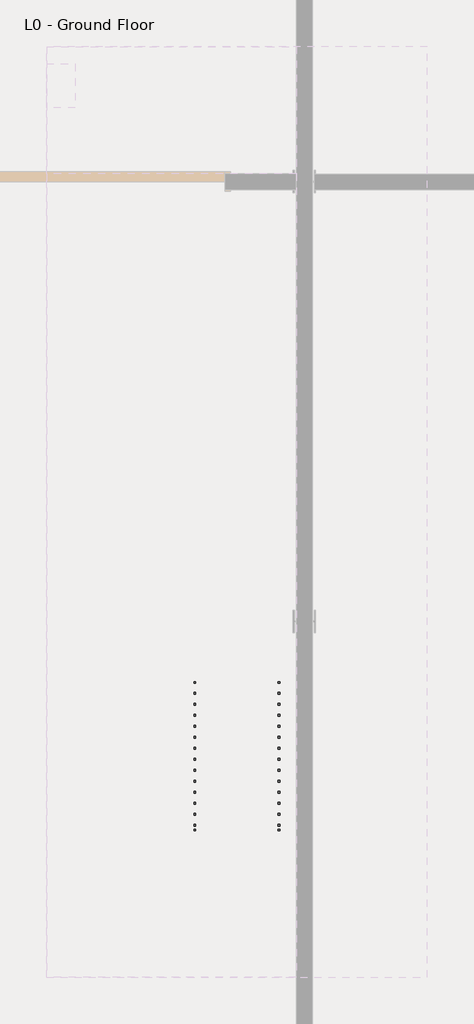
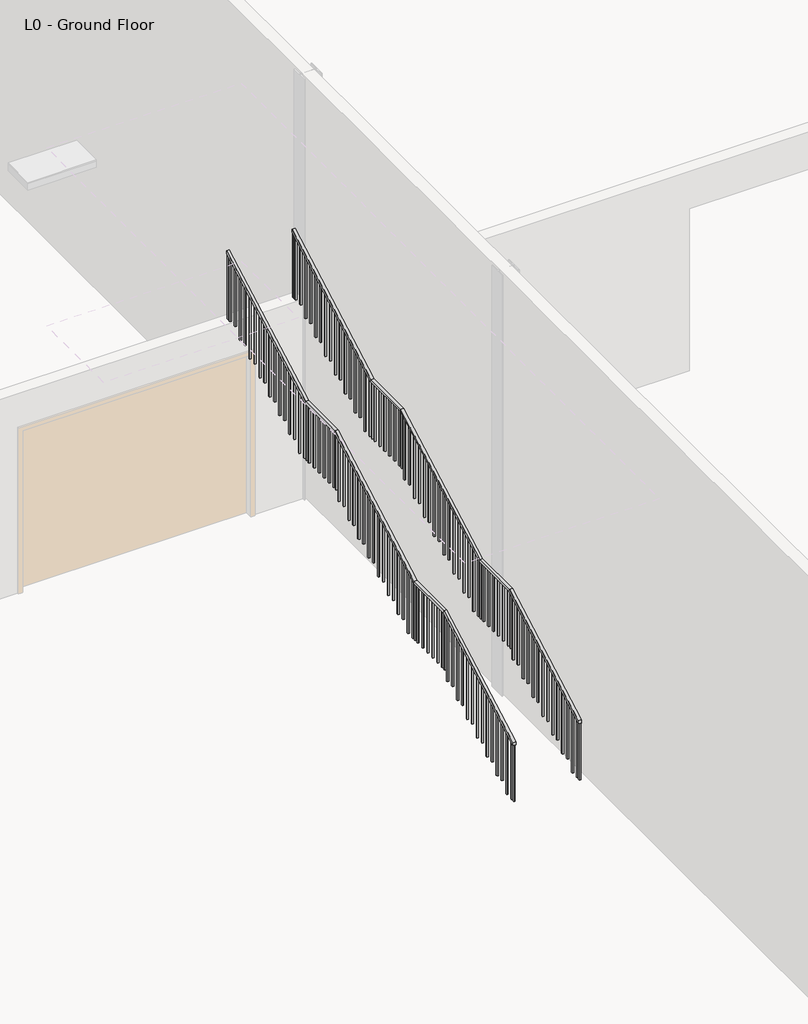
# One storey, part 9 of 14: 2 railings.
"""IFC4 building model written with IfcOpenShell, lengths in millimetres."""

import ifcopenshell
import ifcopenshell.guid

model = None  # the IFC model being written
_history = None  # IfcOwnerHistory: only IFC2X3 demands one
_inside = {}  # id of a spatial element -> (the spatial element, [elements in it])
_under = {}  # id of a project, library or spatial element -> (it, [spatial elements below it])
_declared = {}  # id of a project -> (the project, [libraries it declares])
_typed = {}  # id of a type object -> (the type object, [elements of that type])
_made_of = {}  # id of a material, layer set ... -> (it, [elements and type objects made of it])


def new_model(schema):
    """Start an empty IFC model of exactly this schema.

    Asked for "IFC4X3", IfcOpenShell would pick the latest addendum, in which some entities
    have other attributes; the version numbers below select the first issue.
    IFC2X3 requires an IfcOwnerHistory on every rooted entity: one is made here for all.
    """
    global model, _history
    if schema == "IFC4X3":
        model = ifcopenshell.file(schema_version=(4, 3, 0, 0))
    else:
        model = ifcopenshell.file(schema=schema)
    _inside.clear()
    _under.clear()
    _declared.clear()
    _typed.clear()
    _made_of.clear()
    _history = None
    if model.schema == "IFC2X3":
        org = make("IfcOrganization", Name="unknown")
        user = make(
            "IfcPersonAndOrganization",
            ThePerson=make("IfcPerson", FamilyName="unknown"),
            TheOrganization=org,
        )
        app = make(
            "IfcApplication",
            ApplicationDeveloper=org,
            Version="unknown",
            ApplicationFullName="unknown",
            ApplicationIdentifier="unknown",
        )
        _history = make(
            "IfcOwnerHistory",
            OwningUser=user,
            OwningApplication=app,
            ChangeAction="ADDED",
            CreationDate=0,
        )
    return model


def make(cls, **values):
    """One entity of the class cls with the attributes given. An attribute that is None is left unset."""
    return model.create_entity(
        cls, **{name: value for name, value in values.items() if value is not None}
    )


def rooted(cls, **values):
    """An entity with a GlobalId (a new one), such as an element, a storey or a relation."""
    return make(cls, GlobalId=ifcopenshell.guid.new(), OwnerHistory=_history, **values)


def si_unit(unit_type, name, prefix=None):
    """IfcSIUnit, for example si_unit("LENGTHUNIT", "METRE", prefix="MILLI")."""
    return make("IfcSIUnit", UnitType=unit_type, Prefix=prefix, Name=name)


def assignment(units):
    """IfcUnitAssignment: the units of a project."""
    return None if units is None else make("IfcUnitAssignment", Units=units)


def point(xyz):
    """IfcCartesianPoint."""
    return None if xyz is None else make("IfcCartesianPoint", Coordinates=xyz)


def direction(xyz):
    """IfcDirection."""
    return None if xyz is None else make("IfcDirection", DirectionRatios=xyz)


def frame(location, z_axis=None, x_axis=None):
    """IfcAxis2Placement3D, a coordinate frame: its origin and axes. An axis left out is left unset."""
    return make(
        "IfcAxis2Placement3D",
        Location=point(location),
        Axis=direction(z_axis),
        RefDirection=direction(x_axis),
    )


def origin():
    """The frame at (0, 0, 0) with its axes left unset."""
    return frame((0.0, 0.0, 0.0))


def place(relative_to, where):
    """IfcLocalPlacement: puts the frame where relative to a parent placement (None: the world)."""
    return make(
        "IfcLocalPlacement", PlacementRelTo=relative_to, RelativePlacement=where
    )


def context(
    kind, dimensions, precision=None, world=None, true_north=None, identifier=None
):
    """IfcGeometricRepresentationContext, for example the 3D "Model" context."""
    return make(
        "IfcGeometricRepresentationContext",
        ContextIdentifier=identifier,
        ContextType=kind,
        CoordinateSpaceDimension=dimensions,
        Precision=precision,
        WorldCoordinateSystem=world,
        TrueNorth=true_north,
    )


def project(units=None, contexts=None):
    """IfcProject with its units and contexts."""
    return rooted(
        "IfcProject",
        Name="project",
        RepresentationContexts=contexts,
        UnitsInContext=assignment(units),
    )


def spatial(cls, under=None, at=None, **own):
    """A site, building, storey or space (cls), placed at a placement, below another one or the project."""
    s = rooted(cls, ObjectPlacement=at, **own)
    if under is not None:
        _under.setdefault(under.id(), (under, []))[1].append(s)
    return s


def polyline(points):
    """IfcPolyline through the points."""
    return make("IfcPolyline", Points=[point(p) for p in points])


def outline(outer, holes=None, kind="AREA"):
    """IfcArbitraryClosedProfileDef: a profile drawn as a closed curve; with holes, ...WithVoids."""
    if holes is None:
        return make("IfcArbitraryClosedProfileDef", ProfileType=kind, OuterCurve=outer)
    return make(
        "IfcArbitraryProfileDefWithVoids",
        ProfileType=kind,
        OuterCurve=outer,
        InnerCurves=holes,
    )


def extrude(swept, where, along, depth):
    """IfcExtrudedAreaSolid: the profile swept, set in the frame where, extruded along a direction by depth."""
    return make(
        "IfcExtrudedAreaSolid",
        SweptArea=swept,
        Position=where,
        ExtrudedDirection=direction(along),
        Depth=depth,
    )


def faces_of(points, faces, orient=None, outer=None):
    """IfcFace entities. A face is a list of loops; a loop is a list of indices into points, from 0.

    orient and outer hold one flag for each loop. By default every Orientation is true, the
    first loop of a face is its IfcFaceOuterBound and the others are IfcFaceBound.
    """
    made = []
    for i, loops in enumerate(faces):
        bounds = []
        for j, loop in enumerate(loops):
            is_outer = j == 0 if outer is None else outer[i][j]
            bounds.append(
                make(
                    "IfcFaceOuterBound" if is_outer else "IfcFaceBound",
                    Bound=make("IfcPolyLoop", Polygon=[points[k] for k in loop]),
                    Orientation=True if orient is None else orient[i][j],
                )
            )
        made.append(make("IfcFace", Bounds=bounds))
    return made


def faceted_brep(points, faces, orient=None, outer=None, voids=None):
    """IfcFacetedBrep: a solid bounded by flat faces; with voids (closed shells), ...WithVoids."""
    shared = [point(p) for p in points]
    hull = make("IfcClosedShell", CfsFaces=faces_of(shared, faces, orient, outer))
    if voids is None:
        return make("IfcFacetedBrep", Outer=hull)
    return make(
        "IfcFacetedBrepWithVoids",
        Outer=hull,
        Voids=[
            make(cls, CfsFaces=faces_of(shared, fs, o, b)) for cls, fs, o, b in voids
        ],
    )


def shape(context_of_items, identifier, shape_type, items):
    """IfcShapeRepresentation: the items that make up one representation, for example the "Body"."""
    return make(
        "IfcShapeRepresentation",
        ContextOfItems=context_of_items,
        RepresentationIdentifier=identifier,
        RepresentationType=shape_type,
        Items=items,
    )


def made_of(thing, what):
    """Note that an element or type object is made of a material, layer set ...; save() writes the relation."""
    if what is not None:
        _made_of.setdefault(what.id(), (what, []))[1].append(thing)
    return thing


def element(
    cls,
    number,
    at=None,
    inside=None,
    cuts=None,
    type_object=None,
    material=None,
    context=None,
    identifier="Body",
    shape_type=None,
    held_by="IfcProductDefinitionShape",
    body=None,
    shapes=None,
    **own,
):
    """One element of the class cls, such as IfcWall. Its Tag is "e" and its number.

    at: its placement. inside: the storey or other place that contains it. cuts: it is an
    opening in that element (IfcRelVoidsElement). A single representation is given by context,
    identifier, shape_type and body (its items); several are given by shapes. held_by: the class
    of the entity that holds the representations. save() writes the other relations.
    """
    e = rooted(cls, Tag="e%d" % number, ObjectPlacement=at, **own)
    if body is not None:
        shapes = [shape(context, identifier, shape_type, body)]
    if shapes is not None:
        e.Representation = make(held_by, Representations=shapes)
    if inside is not None:
        _inside.setdefault(inside.id(), (inside, []))[1].append(e)
    if cuts is not None:
        rooted(
            "IfcRelVoidsElement", RelatingBuildingElement=cuts, RelatedOpeningElement=e
        )
    if type_object is not None:
        _typed.setdefault(type_object.id(), (type_object, []))[1].append(e)
    return made_of(e, material)


def aggregate(whole, parts):
    """IfcRelAggregates: a whole, such as a stair, and the parts it consists of."""
    return rooted("IfcRelAggregates", RelatingObject=whole, RelatedObjects=parts)


def save(model, path):
    """Write the relations noted so far, then the file.

    IfcRelAggregates (storeys below a building ...), IfcRelContainedInSpatialStructure (elements
    in a storey), IfcRelDefinesByType, IfcRelAssociatesMaterial and IfcRelDeclares: one each for
    every whole, place, type object, material and project.
    """
    for whole, parts in _under.values():
        aggregate(whole, parts)
    for where, things in _inside.values():
        rooted(
            "IfcRelContainedInSpatialStructure",
            RelatedElements=things,
            RelatingStructure=where,
        )
    for kind, things in _typed.values():
        rooted("IfcRelDefinesByType", RelatedObjects=things, RelatingType=kind)
    for what, things in _made_of.values():
        rooted("IfcRelAssociatesMaterial", RelatedObjects=things, RelatingMaterial=what)
    for by, libraries in _declared.values():
        rooted("IfcRelDeclares", RelatingContext=by, RelatedDefinitions=libraries)
    model.write(path)


model = new_model("IFC4")

# Units and contexts
model_context = context("Model", 3, world=origin())
ifc_project = project(units=[si_unit("LENGTHUNIT", "METRE", prefix="MILLI")], contexts=[model_context])

# Site, building, storey
site = spatial("IfcSite", under=ifc_project)
building = spatial("IfcBuilding", under=site)
storey = spatial("IfcBuildingStorey", under=building, Name="L0 - Ground Floor", Elevation=0.0)

# Railings
placement = place(None, origin())
element("IfcRailing", 1, ObjectType="1100mm", at=placement, inside=storey, context=model_context, shape_type="SolidModel", body=[
    faceted_brep([(10487.9745537, -13916.6257726, 1266.6666667), (10487.9745537, -13916.6257726, 1209.4687214), (10537.9745537, -13916.6257726, 1209.4687214), (10537.9745537, -13916.6257726, 1266.6666667), (10487.9745537, -11816.6257726, 2433.3333333), (10487.9745537, -11803.6694712, 2383.3333333), (10537.9745537, -11803.6694712, 2383.3333333), (10537.9745537, -11816.6257726, 2433.3333333), (10487.9745537, -10916.6257726, 2433.3333333), (10487.9745537, -10903.6694712, 2383.3333333), (10537.9745537, -10903.6694712, 2383.3333333), (10537.9745537, -10916.6257726, 2433.3333333), (10487.9745537, -8516.6257726, 3766.6666667), (10487.9745537, -8503.6694712, 3716.6666667), (10537.9745537, -8503.6694712, 3716.6666667), (10537.9745537, -8516.6257726, 3766.6666667), (10487.9745537, -7616.6257726, 3766.6666667), (10487.9745537, -7603.6694712, 3716.6666667), (10537.9745537, -7603.6694712, 3716.6666667), (10537.9745537, -7616.6257726, 3766.6666667), (10487.9745537, -5216.6257726, 5100.0), (10537.9745537, -5216.6257726, 5100.0), (10537.9745537, -5216.6257726, 5042.8020548), (10487.9745537, -5216.6257726, 5042.8020548)], [[[0, 1, 2, 3]], [[1, 0, 4, 5]], [[2, 1, 5, 6]], [[3, 2, 6, 7]], [[0, 3, 7, 4]], [[5, 4, 8, 9]], [[6, 5, 9, 10]], [[7, 6, 10, 11]], [[4, 7, 11, 8]], [[9, 8, 12, 13]], [[10, 9, 13, 14]], [[11, 10, 14, 15]], [[8, 11, 15, 12]], [[13, 12, 16, 17]], [[14, 13, 17, 18]], [[15, 14, 18, 19]], [[12, 15, 19, 16]], [[20, 21, 22, 23]], [[17, 16, 20, 23]], [[18, 17, 23, 22]], [[19, 18, 22, 21]], [[16, 19, 21, 20]]]),
    extrude(outline(polyline([(-5304.1257726, 3833.3333333), (-5304.1257726, 4994.1909437), (-5279.1257726, 5008.0798326), (-5279.1257726, 3833.3333333), (-5304.1257726, 3833.3333333)])), frame((10500.4745537, 0.0, 0.0), z_axis=(1.0, 0.0, 0.0), x_axis=(0.0, 1.0, 0.0)), (0.0, 0.0, 1.0), 25.0),
    extrude(outline(polyline([(-5454.1257726, 3833.3333333), (-5454.1257726, 4910.8576103), (-5429.1257726, 4924.7464992), (-5429.1257726, 3833.3333333), (-5454.1257726, 3833.3333333)])), frame((10500.4745537, 0.0, 0.0), z_axis=(1.0, 0.0, 0.0), x_axis=(0.0, 1.0, 0.0)), (0.0, 0.0, 1.0), 25.0),
    extrude(outline(polyline([(-5604.1257726, 3666.6666667), (-5604.1257726, 4827.524277), (-5579.1257726, 4841.4131659), (-5579.1257726, 3666.6666667), (-5604.1257726, 3666.6666667)])), frame((10500.4745537, 0.0, 0.0), z_axis=(1.0, 0.0, 0.0), x_axis=(0.0, 1.0, 0.0)), (0.0, 0.0, 1.0), 25.0),
    extrude(outline(polyline([(-5754.1257726, 3666.6666667), (-5754.1257726, 4744.1909437), (-5729.1257726, 4758.0798326), (-5729.1257726, 3666.6666667), (-5754.1257726, 3666.6666667)])), frame((10500.4745537, 0.0, 0.0), z_axis=(1.0, 0.0, 0.0), x_axis=(0.0, 1.0, 0.0)), (0.0, 0.0, 1.0), 25.0),
    extrude(outline(polyline([(-5904.1257726, 3500.0), (-5904.1257726, 4660.8576103), (-5879.1257726, 4674.7464992), (-5879.1257726, 3500.0), (-5904.1257726, 3500.0)])), frame((10500.4745537, 0.0, 0.0), z_axis=(1.0, 0.0, 0.0), x_axis=(0.0, 1.0, 0.0)), (0.0, 0.0, 1.0), 25.0),
    extrude(outline(polyline([(-6054.1257726, 3500.0), (-6054.1257726, 4577.524277), (-6029.1257726, 4591.4131659), (-6029.1257726, 3500.0), (-6054.1257726, 3500.0)])), frame((10500.4745537, 0.0, 0.0), z_axis=(1.0, 0.0, 0.0), x_axis=(0.0, 1.0, 0.0)), (0.0, 0.0, 1.0), 25.0),
    extrude(outline(polyline([(-6204.1257726, 3333.3333333), (-6204.1257726, 4494.1909437), (-6179.1257726, 4508.0798326), (-6179.1257726, 3333.3333333), (-6204.1257726, 3333.3333333)])), frame((10500.4745537, 0.0, 0.0), z_axis=(1.0, 0.0, 0.0), x_axis=(0.0, 1.0, 0.0)), (0.0, 0.0, 1.0), 25.0),
    extrude(outline(polyline([(-6354.1257726, 3333.3333333), (-6354.1257726, 4410.8576103), (-6329.1257726, 4424.7464992), (-6329.1257726, 3333.3333333), (-6354.1257726, 3333.3333333)])), frame((10500.4745537, 0.0, 0.0), z_axis=(1.0, 0.0, 0.0), x_axis=(0.0, 1.0, 0.0)), (0.0, 0.0, 1.0), 25.0),
    extrude(outline(polyline([(-6504.1257726, 3166.6666667), (-6504.1257726, 4327.524277), (-6479.1257726, 4341.4131659), (-6479.1257726, 3166.6666667), (-6504.1257726, 3166.6666667)])), frame((10500.4745537, 0.0, 0.0), z_axis=(1.0, 0.0, 0.0), x_axis=(0.0, 1.0, 0.0)), (0.0, 0.0, 1.0), 25.0),
    extrude(outline(polyline([(-6654.1257726, 3166.6666667), (-6654.1257726, 4244.1909437), (-6629.1257726, 4258.0798326), (-6629.1257726, 3166.6666667), (-6654.1257726, 3166.6666667)])), frame((10500.4745537, 0.0, 0.0), z_axis=(1.0, 0.0, 0.0), x_axis=(0.0, 1.0, 0.0)), (0.0, 0.0, 1.0), 25.0),
    extrude(outline(polyline([(-6804.1257726, 3000.0), (-6804.1257726, 4160.8576103), (-6779.1257726, 4174.7464992), (-6779.1257726, 3000.0), (-6804.1257726, 3000.0)])), frame((10500.4745537, 0.0, 0.0), z_axis=(1.0, 0.0, 0.0), x_axis=(0.0, 1.0, 0.0)), (0.0, 0.0, 1.0), 25.0),
    extrude(outline(polyline([(-6954.1257726, 3000.0), (-6954.1257726, 4077.524277), (-6929.1257726, 4091.4131659), (-6929.1257726, 3000.0), (-6954.1257726, 3000.0)])), frame((10500.4745537, 0.0, 0.0), z_axis=(1.0, 0.0, 0.0), x_axis=(0.0, 1.0, 0.0)), (0.0, 0.0, 1.0), 25.0),
    extrude(outline(polyline([(-7104.1257726, 2833.3333333), (-7104.1257726, 3994.1909437), (-7079.1257726, 4008.0798326), (-7079.1257726, 2833.3333333), (-7104.1257726, 2833.3333333)])), frame((10500.4745537, 0.0, 0.0), z_axis=(1.0, 0.0, 0.0), x_axis=(0.0, 1.0, 0.0)), (0.0, 0.0, 1.0), 25.0),
    extrude(outline(polyline([(-7254.1257726, 2833.3333333), (-7254.1257726, 3910.8576103), (-7229.1257726, 3924.7464992), (-7229.1257726, 2833.3333333), (-7254.1257726, 2833.3333333)])), frame((10500.4745537, 0.0, 0.0), z_axis=(1.0, 0.0, 0.0), x_axis=(0.0, 1.0, 0.0)), (0.0, 0.0, 1.0), 25.0),
    extrude(outline(polyline([(-7404.1257726, 2666.6666667), (-7404.1257726, 3827.524277), (-7379.1257726, 3841.4131659), (-7379.1257726, 2666.6666667), (-7404.1257726, 2666.6666667)])), frame((10500.4745537, 0.0, 0.0), z_axis=(1.0, 0.0, 0.0), x_axis=(0.0, 1.0, 0.0)), (0.0, 0.0, 1.0), 25.0),
    extrude(outline(polyline([(-7554.1257726, 2666.6666667), (-7554.1257726, 3744.1909437), (-7529.1257726, 3758.0798326), (-7529.1257726, 2666.6666667), (-7554.1257726, 2666.6666667)])), frame((10500.4745537, 0.0, 0.0), z_axis=(1.0, 0.0, 0.0), x_axis=(0.0, 1.0, 0.0)), (0.0, 0.0, 1.0), 25.0),
    extrude(outline(polyline([(10525.4745537, -7704.1257726), (10500.4745537, -7704.1257726), (10500.4745537, -7679.1257726), (10525.4745537, -7679.1257726), (10525.4745537, -7704.1257726)])), frame((0.0, 0.0, 2666.6666667), z_axis=(0.0, 0.0, 1.0), x_axis=(1.0, 0.0, 0.0)), (0.0, 0.0, 1.0), 1050.0),
    extrude(outline(polyline([(10525.4745537, -7854.1257726), (10500.4745537, -7854.1257726), (10500.4745537, -7829.1257726), (10525.4745537, -7829.1257726), (10525.4745537, -7854.1257726)])), frame((0.0, 0.0, 2666.6666667), z_axis=(0.0, 0.0, 1.0), x_axis=(1.0, 0.0, 0.0)), (0.0, 0.0, 1.0), 1050.0),
    extrude(outline(polyline([(10525.4745537, -8004.1257726), (10500.4745537, -8004.1257726), (10500.4745537, -7979.1257726), (10525.4745537, -7979.1257726), (10525.4745537, -8004.1257726)])), frame((0.0, 0.0, 2666.6666667), z_axis=(0.0, 0.0, 1.0), x_axis=(1.0, 0.0, 0.0)), (0.0, 0.0, 1.0), 1050.0),
    extrude(outline(polyline([(10525.4745537, -8154.1257726), (10500.4745537, -8154.1257726), (10500.4745537, -8129.1257726), (10525.4745537, -8129.1257726), (10525.4745537, -8154.1257726)])), frame((0.0, 0.0, 2666.6666667), z_axis=(0.0, 0.0, 1.0), x_axis=(1.0, 0.0, 0.0)), (0.0, 0.0, 1.0), 1050.0),
    extrude(outline(polyline([(10525.4745537, -8304.1257726), (10500.4745537, -8304.1257726), (10500.4745537, -8279.1257726), (10525.4745537, -8279.1257726), (10525.4745537, -8304.1257726)])), frame((0.0, 0.0, 2666.6666667), z_axis=(0.0, 0.0, 1.0), x_axis=(1.0, 0.0, 0.0)), (0.0, 0.0, 1.0), 1050.0),
    extrude(outline(polyline([(10525.4745537, -8454.1257726), (10500.4745537, -8454.1257726), (10500.4745537, -8429.1257726), (10525.4745537, -8429.1257726), (10525.4745537, -8454.1257726)])), frame((0.0, 0.0, 2666.6666667), z_axis=(0.0, 0.0, 1.0), x_axis=(1.0, 0.0, 0.0)), (0.0, 0.0, 1.0), 1050.0),
    extrude(outline(polyline([(-8604.1257726, 2500.0), (-8604.1257726, 3660.8576103), (-8579.1257726, 3674.7464992), (-8579.1257726, 2500.0), (-8604.1257726, 2500.0)])), frame((10500.4745537, 0.0, 0.0), z_axis=(1.0, 0.0, 0.0), x_axis=(0.0, 1.0, 0.0)), (0.0, 0.0, 1.0), 25.0),
    extrude(outline(polyline([(-8754.1257726, 2500.0), (-8754.1257726, 3577.524277), (-8729.1257726, 3591.4131659), (-8729.1257726, 2500.0), (-8754.1257726, 2500.0)])), frame((10500.4745537, 0.0, 0.0), z_axis=(1.0, 0.0, 0.0), x_axis=(0.0, 1.0, 0.0)), (0.0, 0.0, 1.0), 25.0),
    extrude(outline(polyline([(-8904.1257726, 2333.3333333), (-8904.1257726, 3494.1909437), (-8879.1257726, 3508.0798326), (-8879.1257726, 2333.3333333), (-8904.1257726, 2333.3333333)])), frame((10500.4745537, 0.0, 0.0), z_axis=(1.0, 0.0, 0.0), x_axis=(0.0, 1.0, 0.0)), (0.0, 0.0, 1.0), 25.0),
    extrude(outline(polyline([(-9054.1257726, 2333.3333333), (-9054.1257726, 3410.8576103), (-9029.1257726, 3424.7464992), (-9029.1257726, 2333.3333333), (-9054.1257726, 2333.3333333)])), frame((10500.4745537, 0.0, 0.0), z_axis=(1.0, 0.0, 0.0), x_axis=(0.0, 1.0, 0.0)), (0.0, 0.0, 1.0), 25.0),
    extrude(outline(polyline([(-9204.1257726, 2166.6666667), (-9204.1257726, 3327.524277), (-9179.1257726, 3341.4131659), (-9179.1257726, 2166.6666667), (-9204.1257726, 2166.6666667)])), frame((10500.4745537, 0.0, 0.0), z_axis=(1.0, 0.0, 0.0), x_axis=(0.0, 1.0, 0.0)), (0.0, 0.0, 1.0), 25.0),
    extrude(outline(polyline([(-9354.1257726, 2166.6666667), (-9354.1257726, 3244.1909437), (-9329.1257726, 3258.0798326), (-9329.1257726, 2166.6666667), (-9354.1257726, 2166.6666667)])), frame((10500.4745537, 0.0, 0.0), z_axis=(1.0, 0.0, 0.0), x_axis=(0.0, 1.0, 0.0)), (0.0, 0.0, 1.0), 25.0),
    extrude(outline(polyline([(-9504.1257726, 2000.0), (-9504.1257726, 3160.8576103), (-9479.1257726, 3174.7464992), (-9479.1257726, 2000.0), (-9504.1257726, 2000.0)])), frame((10500.4745537, 0.0, 0.0), z_axis=(1.0, 0.0, 0.0), x_axis=(0.0, 1.0, 0.0)), (0.0, 0.0, 1.0), 25.0),
    extrude(outline(polyline([(-9654.1257726, 2000.0), (-9654.1257726, 3077.524277), (-9629.1257726, 3091.4131659), (-9629.1257726, 2000.0), (-9654.1257726, 2000.0)])), frame((10500.4745537, 0.0, 0.0), z_axis=(1.0, 0.0, 0.0), x_axis=(0.0, 1.0, 0.0)), (0.0, 0.0, 1.0), 25.0),
    extrude(outline(polyline([(-9804.1257726, 1833.3333333), (-9804.1257726, 2994.1909437), (-9779.1257726, 3008.0798326), (-9779.1257726, 1833.3333333), (-9804.1257726, 1833.3333333)])), frame((10500.4745537, 0.0, 0.0), z_axis=(1.0, 0.0, 0.0), x_axis=(0.0, 1.0, 0.0)), (0.0, 0.0, 1.0), 25.0),
    extrude(outline(polyline([(-9954.1257726, 1833.3333333), (-9954.1257726, 2910.8576103), (-9929.1257726, 2924.7464992), (-9929.1257726, 1833.3333333), (-9954.1257726, 1833.3333333)])), frame((10500.4745537, 0.0, 0.0), z_axis=(1.0, 0.0, 0.0), x_axis=(0.0, 1.0, 0.0)), (0.0, 0.0, 1.0), 25.0),
    extrude(outline(polyline([(-10104.1257726, 1666.6666667), (-10104.1257726, 2827.524277), (-10079.1257726, 2841.4131659), (-10079.1257726, 1666.6666667), (-10104.1257726, 1666.6666667)])), frame((10500.4745537, 0.0, 0.0), z_axis=(1.0, 0.0, 0.0), x_axis=(0.0, 1.0, 0.0)), (0.0, 0.0, 1.0), 25.0),
    extrude(outline(polyline([(-10254.1257726, 1666.6666667), (-10254.1257726, 2744.1909437), (-10229.1257726, 2758.0798326), (-10229.1257726, 1666.6666667), (-10254.1257726, 1666.6666667)])), frame((10500.4745537, 0.0, 0.0), z_axis=(1.0, 0.0, 0.0), x_axis=(0.0, 1.0, 0.0)), (0.0, 0.0, 1.0), 25.0),
    extrude(outline(polyline([(-10404.1257726, 1500.0), (-10404.1257726, 2660.8576103), (-10379.1257726, 2674.7464992), (-10379.1257726, 1500.0), (-10404.1257726, 1500.0)])), frame((10500.4745537, 0.0, 0.0), z_axis=(1.0, 0.0, 0.0), x_axis=(0.0, 1.0, 0.0)), (0.0, 0.0, 1.0), 25.0),
    extrude(outline(polyline([(-10554.1257726, 1500.0), (-10554.1257726, 2577.524277), (-10529.1257726, 2591.4131659), (-10529.1257726, 1500.0), (-10554.1257726, 1500.0)])), frame((10500.4745537, 0.0, 0.0), z_axis=(1.0, 0.0, 0.0), x_axis=(0.0, 1.0, 0.0)), (0.0, 0.0, 1.0), 25.0),
    extrude(outline(polyline([(-10704.1257726, 1333.3333333), (-10704.1257726, 2494.1909437), (-10679.1257726, 2508.0798326), (-10679.1257726, 1333.3333333), (-10704.1257726, 1333.3333333)])), frame((10500.4745537, 0.0, 0.0), z_axis=(1.0, 0.0, 0.0), x_axis=(0.0, 1.0, 0.0)), (0.0, 0.0, 1.0), 25.0),
    extrude(outline(polyline([(-10854.1257726, 1333.3333333), (-10854.1257726, 2410.8576103), (-10829.1257726, 2424.7464992), (-10829.1257726, 1333.3333333), (-10854.1257726, 1333.3333333)])), frame((10500.4745537, 0.0, 0.0), z_axis=(1.0, 0.0, 0.0), x_axis=(0.0, 1.0, 0.0)), (0.0, 0.0, 1.0), 25.0),
    extrude(outline(polyline([(10525.4745537, -11004.1257726), (10500.4745537, -11004.1257726), (10500.4745537, -10979.1257726), (10525.4745537, -10979.1257726), (10525.4745537, -11004.1257726)])), frame((0.0, 0.0, 1333.3333333), z_axis=(0.0, 0.0, 1.0), x_axis=(1.0, 0.0, 0.0)), (0.0, 0.0, 1.0), 1050.0),
    extrude(outline(polyline([(10525.4745537, -11154.1257726), (10500.4745537, -11154.1257726), (10500.4745537, -11129.1257726), (10525.4745537, -11129.1257726), (10525.4745537, -11154.1257726)])), frame((0.0, 0.0, 1333.3333333), z_axis=(0.0, 0.0, 1.0), x_axis=(1.0, 0.0, 0.0)), (0.0, 0.0, 1.0), 1050.0),
    extrude(outline(polyline([(10525.4745537, -11304.1257726), (10500.4745537, -11304.1257726), (10500.4745537, -11279.1257726), (10525.4745537, -11279.1257726), (10525.4745537, -11304.1257726)])), frame((0.0, 0.0, 1333.3333333), z_axis=(0.0, 0.0, 1.0), x_axis=(1.0, 0.0, 0.0)), (0.0, 0.0, 1.0), 1050.0),
    extrude(outline(polyline([(10525.4745537, -11454.1257726), (10500.4745537, -11454.1257726), (10500.4745537, -11429.1257726), (10525.4745537, -11429.1257726), (10525.4745537, -11454.1257726)])), frame((0.0, 0.0, 1333.3333333), z_axis=(0.0, 0.0, 1.0), x_axis=(1.0, 0.0, 0.0)), (0.0, 0.0, 1.0), 1050.0),
    extrude(outline(polyline([(10525.4745537, -11604.1257726), (10500.4745537, -11604.1257726), (10500.4745537, -11579.1257726), (10525.4745537, -11579.1257726), (10525.4745537, -11604.1257726)])), frame((0.0, 0.0, 1333.3333333), z_axis=(0.0, 0.0, 1.0), x_axis=(1.0, 0.0, 0.0)), (0.0, 0.0, 1.0), 1050.0),
    extrude(outline(polyline([(10525.4745537, -11754.1257726), (10500.4745537, -11754.1257726), (10500.4745537, -11729.1257726), (10525.4745537, -11729.1257726), (10525.4745537, -11754.1257726)])), frame((0.0, 0.0, 1333.3333333), z_axis=(0.0, 0.0, 1.0), x_axis=(1.0, 0.0, 0.0)), (0.0, 0.0, 1.0), 1050.0),
    extrude(outline(polyline([(-11904.1257726, 1166.6666667), (-11904.1257726, 2327.524277), (-11879.1257726, 2341.4131659), (-11879.1257726, 1166.6666667), (-11904.1257726, 1166.6666667)])), frame((10500.4745537, 0.0, 0.0), z_axis=(1.0, 0.0, 0.0), x_axis=(0.0, 1.0, 0.0)), (0.0, 0.0, 1.0), 25.0),
    extrude(outline(polyline([(-12054.1257726, 1166.6666667), (-12054.1257726, 2244.1909437), (-12029.1257726, 2258.0798326), (-12029.1257726, 1166.6666667), (-12054.1257726, 1166.6666667)])), frame((10500.4745537, 0.0, 0.0), z_axis=(1.0, 0.0, 0.0), x_axis=(0.0, 1.0, 0.0)), (0.0, 0.0, 1.0), 25.0),
    extrude(outline(polyline([(-12204.1257726, 1000.0), (-12204.1257726, 2160.8576103), (-12179.1257726, 2174.7464992), (-12179.1257726, 1000.0), (-12204.1257726, 1000.0)])), frame((10500.4745537, 0.0, 0.0), z_axis=(1.0, 0.0, 0.0), x_axis=(0.0, 1.0, 0.0)), (0.0, 0.0, 1.0), 25.0),
    extrude(outline(polyline([(-12354.1257726, 1000.0), (-12354.1257726, 2077.524277), (-12329.1257726, 2091.4131659), (-12329.1257726, 1000.0), (-12354.1257726, 1000.0)])), frame((10500.4745537, 0.0, 0.0), z_axis=(1.0, 0.0, 0.0), x_axis=(0.0, 1.0, 0.0)), (0.0, 0.0, 1.0), 25.0),
    extrude(outline(polyline([(-12504.1257726, 833.3333333), (-12504.1257726, 1994.1909437), (-12479.1257726, 2008.0798326), (-12479.1257726, 833.3333333), (-12504.1257726, 833.3333333)])), frame((10500.4745537, 0.0, 0.0), z_axis=(1.0, 0.0, 0.0), x_axis=(0.0, 1.0, 0.0)), (0.0, 0.0, 1.0), 25.0),
    extrude(outline(polyline([(-12654.1257726, 833.3333333), (-12654.1257726, 1910.8576103), (-12629.1257726, 1924.7464992), (-12629.1257726, 833.3333333), (-12654.1257726, 833.3333333)])), frame((10500.4745537, 0.0, 0.0), z_axis=(1.0, 0.0, 0.0), x_axis=(0.0, 1.0, 0.0)), (0.0, 0.0, 1.0), 25.0),
    extrude(outline(polyline([(-12804.1257726, 666.6666667), (-12804.1257726, 1827.524277), (-12779.1257726, 1841.4131659), (-12779.1257726, 666.6666667), (-12804.1257726, 666.6666667)])), frame((10500.4745537, 0.0, 0.0), z_axis=(1.0, 0.0, 0.0), x_axis=(0.0, 1.0, 0.0)), (0.0, 0.0, 1.0), 25.0),
    extrude(outline(polyline([(-12954.1257726, 666.6666667), (-12954.1257726, 1744.1909437), (-12929.1257726, 1758.0798326), (-12929.1257726, 666.6666667), (-12954.1257726, 666.6666667)])), frame((10500.4745537, 0.0, 0.0), z_axis=(1.0, 0.0, 0.0), x_axis=(0.0, 1.0, 0.0)), (0.0, 0.0, 1.0), 25.0),
    extrude(outline(polyline([(-13104.1257726, 500.0), (-13104.1257726, 1660.8576103), (-13079.1257726, 1674.7464992), (-13079.1257726, 500.0), (-13104.1257726, 500.0)])), frame((10500.4745537, 0.0, 0.0), z_axis=(1.0, 0.0, 0.0), x_axis=(0.0, 1.0, 0.0)), (0.0, 0.0, 1.0), 25.0),
    extrude(outline(polyline([(-13254.1257726, 500.0), (-13254.1257726, 1577.524277), (-13229.1257726, 1591.4131659), (-13229.1257726, 500.0), (-13254.1257726, 500.0)])), frame((10500.4745537, 0.0, 0.0), z_axis=(1.0, 0.0, 0.0), x_axis=(0.0, 1.0, 0.0)), (0.0, 0.0, 1.0), 25.0),
    extrude(outline(polyline([(-13404.1257726, 333.3333333), (-13404.1257726, 1494.1909437), (-13379.1257726, 1508.0798326), (-13379.1257726, 333.3333333), (-13404.1257726, 333.3333333)])), frame((10500.4745537, 0.0, 0.0), z_axis=(1.0, 0.0, 0.0), x_axis=(0.0, 1.0, 0.0)), (0.0, 0.0, 1.0), 25.0),
    extrude(outline(polyline([(-13554.1257726, 333.3333333), (-13554.1257726, 1410.8576103), (-13529.1257726, 1424.7464992), (-13529.1257726, 333.3333333), (-13554.1257726, 333.3333333)])), frame((10500.4745537, 0.0, 0.0), z_axis=(1.0, 0.0, 0.0), x_axis=(0.0, 1.0, 0.0)), (0.0, 0.0, 1.0), 25.0),
    extrude(outline(polyline([(-13704.1257726, 166.6666667), (-13704.1257726, 1327.524277), (-13679.1257726, 1341.4131659), (-13679.1257726, 166.6666667), (-13704.1257726, 166.6666667)])), frame((10500.4745537, 0.0, 0.0), z_axis=(1.0, 0.0, 0.0), x_axis=(0.0, 1.0, 0.0)), (0.0, 0.0, 1.0), 25.0),
    extrude(outline(polyline([(-13854.1257726, 166.6666667), (-13854.1257726, 1244.1909437), (-13829.1257726, 1258.0798326), (-13829.1257726, 166.6666667), (-13854.1257726, 166.6666667)])), frame((10500.4745537, 0.0, 0.0), z_axis=(1.0, 0.0, 0.0), x_axis=(0.0, 1.0, 0.0)), (0.0, 0.0, 1.0), 25.0),
    extrude(outline(polyline([(10525.4745537, -7629.1257726), (10500.4745537, -7629.1257726), (10500.4745537, -7604.1257726), (10525.4745537, -7604.1257726), (10525.4745537, -7629.1257726)])), frame((0.0, 0.0, 2666.6666667), z_axis=(0.0, 0.0, 1.0), x_axis=(1.0, 0.0, 0.0)), (0.0, 0.0, 1.0), 1050.0),
    extrude(outline(polyline([(-8529.1257726, 2666.6666667), (-8529.1257726, 3702.524277), (-8504.1257726, 3716.4131659), (-8504.1257726, 2666.6666667), (-8529.1257726, 2666.6666667)])), frame((10500.4745537, 0.0, 0.0), z_axis=(1.0, 0.0, 0.0), x_axis=(0.0, 1.0, 0.0)), (0.0, 0.0, 1.0), 25.0),
    extrude(outline(polyline([(10525.4745537, -10929.1257726), (10500.4745537, -10929.1257726), (10500.4745537, -10904.1257726), (10525.4745537, -10904.1257726), (10525.4745537, -10929.1257726)])), frame((0.0, 0.0, 1333.3333333), z_axis=(0.0, 0.0, 1.0), x_axis=(1.0, 0.0, 0.0)), (0.0, 0.0, 1.0), 1050.0),
    extrude(outline(polyline([(-11829.1257726, 1333.3333333), (-11829.1257726, 2369.1909437), (-11804.1257726, 2383.0798326), (-11804.1257726, 1333.3333333), (-11829.1257726, 1333.3333333)])), frame((10500.4745537, 0.0, 0.0), z_axis=(1.0, 0.0, 0.0), x_axis=(0.0, 1.0, 0.0)), (0.0, 0.0, 1.0), 25.0),
    extrude(outline(polyline([(-5241.6257726, 3833.3333333), (-5241.6257726, 5028.9131659), (-5216.6257726, 5042.8020548), (-5216.6257726, 3833.3333333), (-5241.6257726, 3833.3333333)])), frame((10500.4745537, 0.0, 0.0), z_axis=(1.0, 0.0, 0.0), x_axis=(0.0, 1.0, 0.0)), (0.0, 0.0, 1.0), 25.0),
    extrude(outline(polyline([(-13916.6257726, 166.6666667), (-13916.6257726, 1209.4687214), (-13891.6257726, 1223.3576103), (-13891.6257726, 166.6666667), (-13916.6257726, 166.6666667)])), frame((10500.4745537, 0.0, 0.0), z_axis=(1.0, 0.0, 0.0), x_axis=(0.0, 1.0, 0.0)), (0.0, 0.0, 1.0), 25.0),
])
element("IfcRailing", 2, ObjectType="1100mm", at=placement, inside=storey, context=model_context, shape_type="SolidModel", body=[
    faceted_brep([(9338.7745537, -13916.6257726, 1266.6666667), (9338.7745537, -13916.6257726, 1209.4687214), (9388.7745537, -13916.6257726, 1209.4687214), (9388.7745537, -13916.6257726, 1266.6666667), (9338.7745537, -11816.6257726, 2433.3333333), (9338.7745537, -11803.6694712, 2383.3333333), (9388.7745537, -11803.6694712, 2383.3333333), (9388.7745537, -11816.6257726, 2433.3333333), (9338.7745537, -10916.6257726, 2433.3333333), (9338.7745537, -10903.6694712, 2383.3333333), (9388.7745537, -10903.6694712, 2383.3333333), (9388.7745537, -10916.6257726, 2433.3333333), (9338.7745537, -8516.6257726, 3766.6666667), (9338.7745537, -8503.6694712, 3716.6666667), (9388.7745537, -8503.6694712, 3716.6666667), (9388.7745537, -8516.6257726, 3766.6666667), (9338.7745537, -7616.6257726, 3766.6666667), (9338.7745537, -7603.6694712, 3716.6666667), (9388.7745537, -7603.6694712, 3716.6666667), (9388.7745537, -7616.6257726, 3766.6666667), (9338.7745537, -5216.6257726, 5100.0), (9388.7745537, -5216.6257726, 5100.0), (9388.7745537, -5216.6257726, 5042.8020548), (9338.7745537, -5216.6257726, 5042.8020548)], [[[0, 1, 2, 3]], [[1, 0, 4, 5]], [[2, 1, 5, 6]], [[3, 2, 6, 7]], [[0, 3, 7, 4]], [[5, 4, 8, 9]], [[6, 5, 9, 10]], [[7, 6, 10, 11]], [[4, 7, 11, 8]], [[9, 8, 12, 13]], [[10, 9, 13, 14]], [[11, 10, 14, 15]], [[8, 11, 15, 12]], [[13, 12, 16, 17]], [[14, 13, 17, 18]], [[15, 14, 18, 19]], [[12, 15, 19, 16]], [[20, 21, 22, 23]], [[17, 16, 20, 23]], [[18, 17, 23, 22]], [[19, 18, 22, 21]], [[16, 19, 21, 20]]]),
    extrude(outline(polyline([(-5304.1257726, 4994.1909437), (-5279.1257726, 5008.0798326), (-5279.1257726, 3833.3333333), (-5304.1257726, 3833.3333333), (-5304.1257726, 4994.1909437)])), frame((9351.2745537, 0.0, 0.0), z_axis=(1.0, 0.0, 0.0), x_axis=(0.0, 1.0, 0.0)), (0.0, 0.0, 1.0), 25.0),
    extrude(outline(polyline([(-5454.1257726, 4910.8576103), (-5429.1257726, 4924.7464992), (-5429.1257726, 3833.3333333), (-5454.1257726, 3833.3333333), (-5454.1257726, 4910.8576103)])), frame((9351.2745537, 0.0, 0.0), z_axis=(1.0, 0.0, 0.0), x_axis=(0.0, 1.0, 0.0)), (0.0, 0.0, 1.0), 25.0),
    extrude(outline(polyline([(-5604.1257726, 4827.524277), (-5579.1257726, 4841.4131659), (-5579.1257726, 3666.6666667), (-5604.1257726, 3666.6666667), (-5604.1257726, 4827.524277)])), frame((9351.2745537, 0.0, 0.0), z_axis=(1.0, 0.0, 0.0), x_axis=(0.0, 1.0, 0.0)), (0.0, 0.0, 1.0), 25.0),
    extrude(outline(polyline([(-5754.1257726, 4744.1909437), (-5729.1257726, 4758.0798326), (-5729.1257726, 3666.6666667), (-5754.1257726, 3666.6666667), (-5754.1257726, 4744.1909437)])), frame((9351.2745537, 0.0, 0.0), z_axis=(1.0, 0.0, 0.0), x_axis=(0.0, 1.0, 0.0)), (0.0, 0.0, 1.0), 25.0),
    extrude(outline(polyline([(-5904.1257726, 4660.8576103), (-5879.1257726, 4674.7464992), (-5879.1257726, 3500.0), (-5904.1257726, 3500.0), (-5904.1257726, 4660.8576103)])), frame((9351.2745537, 0.0, 0.0), z_axis=(1.0, 0.0, 0.0), x_axis=(0.0, 1.0, 0.0)), (0.0, 0.0, 1.0), 25.0),
    extrude(outline(polyline([(-6054.1257726, 4577.524277), (-6029.1257726, 4591.4131659), (-6029.1257726, 3500.0), (-6054.1257726, 3500.0), (-6054.1257726, 4577.524277)])), frame((9351.2745537, 0.0, 0.0), z_axis=(1.0, 0.0, 0.0), x_axis=(0.0, 1.0, 0.0)), (0.0, 0.0, 1.0), 25.0),
    extrude(outline(polyline([(-6204.1257726, 4494.1909437), (-6179.1257726, 4508.0798326), (-6179.1257726, 3333.3333333), (-6204.1257726, 3333.3333333), (-6204.1257726, 4494.1909437)])), frame((9351.2745537, 0.0, 0.0), z_axis=(1.0, 0.0, 0.0), x_axis=(0.0, 1.0, 0.0)), (0.0, 0.0, 1.0), 25.0),
    extrude(outline(polyline([(-6354.1257726, 4410.8576103), (-6329.1257726, 4424.7464992), (-6329.1257726, 3333.3333333), (-6354.1257726, 3333.3333333), (-6354.1257726, 4410.8576103)])), frame((9351.2745537, 0.0, 0.0), z_axis=(1.0, 0.0, 0.0), x_axis=(0.0, 1.0, 0.0)), (0.0, 0.0, 1.0), 25.0),
    extrude(outline(polyline([(-6504.1257726, 4327.524277), (-6479.1257726, 4341.4131659), (-6479.1257726, 3166.6666667), (-6504.1257726, 3166.6666667), (-6504.1257726, 4327.524277)])), frame((9351.2745537, 0.0, 0.0), z_axis=(1.0, 0.0, 0.0), x_axis=(0.0, 1.0, 0.0)), (0.0, 0.0, 1.0), 25.0),
    extrude(outline(polyline([(-6654.1257726, 4244.1909437), (-6629.1257726, 4258.0798326), (-6629.1257726, 3166.6666667), (-6654.1257726, 3166.6666667), (-6654.1257726, 4244.1909437)])), frame((9351.2745537, 0.0, 0.0), z_axis=(1.0, 0.0, 0.0), x_axis=(0.0, 1.0, 0.0)), (0.0, 0.0, 1.0), 25.0),
    extrude(outline(polyline([(-6804.1257726, 4160.8576103), (-6779.1257726, 4174.7464992), (-6779.1257726, 3000.0), (-6804.1257726, 3000.0), (-6804.1257726, 4160.8576103)])), frame((9351.2745537, 0.0, 0.0), z_axis=(1.0, 0.0, 0.0), x_axis=(0.0, 1.0, 0.0)), (0.0, 0.0, 1.0), 25.0),
    extrude(outline(polyline([(-6954.1257726, 4077.524277), (-6929.1257726, 4091.4131659), (-6929.1257726, 3000.0), (-6954.1257726, 3000.0), (-6954.1257726, 4077.524277)])), frame((9351.2745537, 0.0, 0.0), z_axis=(1.0, 0.0, 0.0), x_axis=(0.0, 1.0, 0.0)), (0.0, 0.0, 1.0), 25.0),
    extrude(outline(polyline([(-7104.1257726, 3994.1909437), (-7079.1257726, 4008.0798326), (-7079.1257726, 2833.3333333), (-7104.1257726, 2833.3333333), (-7104.1257726, 3994.1909437)])), frame((9351.2745537, 0.0, 0.0), z_axis=(1.0, 0.0, 0.0), x_axis=(0.0, 1.0, 0.0)), (0.0, 0.0, 1.0), 25.0),
    extrude(outline(polyline([(-7254.1257726, 3910.8576103), (-7229.1257726, 3924.7464992), (-7229.1257726, 2833.3333333), (-7254.1257726, 2833.3333333), (-7254.1257726, 3910.8576103)])), frame((9351.2745537, 0.0, 0.0), z_axis=(1.0, 0.0, 0.0), x_axis=(0.0, 1.0, 0.0)), (0.0, 0.0, 1.0), 25.0),
    extrude(outline(polyline([(-7404.1257726, 3827.524277), (-7379.1257726, 3841.4131659), (-7379.1257726, 2666.6666667), (-7404.1257726, 2666.6666667), (-7404.1257726, 3827.524277)])), frame((9351.2745537, 0.0, 0.0), z_axis=(1.0, 0.0, 0.0), x_axis=(0.0, 1.0, 0.0)), (0.0, 0.0, 1.0), 25.0),
    extrude(outline(polyline([(-7554.1257726, 3744.1909437), (-7529.1257726, 3758.0798326), (-7529.1257726, 2666.6666667), (-7554.1257726, 2666.6666667), (-7554.1257726, 3744.1909437)])), frame((9351.2745537, 0.0, 0.0), z_axis=(1.0, 0.0, 0.0), x_axis=(0.0, 1.0, 0.0)), (0.0, 0.0, 1.0), 25.0),
    extrude(outline(polyline([(9351.2745537, -7704.1257726), (9351.2745537, -7679.1257726), (9376.2745537, -7679.1257726), (9376.2745537, -7704.1257726), (9351.2745537, -7704.1257726)])), frame((0.0, 0.0, 2666.6666667), z_axis=(0.0, 0.0, 1.0), x_axis=(1.0, 0.0, 0.0)), (0.0, 0.0, 1.0), 1050.0),
    extrude(outline(polyline([(9351.2745537, -7854.1257726), (9351.2745537, -7829.1257726), (9376.2745537, -7829.1257726), (9376.2745537, -7854.1257726), (9351.2745537, -7854.1257726)])), frame((0.0, 0.0, 2666.6666667), z_axis=(0.0, 0.0, 1.0), x_axis=(1.0, 0.0, 0.0)), (0.0, 0.0, 1.0), 1050.0),
    extrude(outline(polyline([(9351.2745537, -8004.1257726), (9351.2745537, -7979.1257726), (9376.2745537, -7979.1257726), (9376.2745537, -8004.1257726), (9351.2745537, -8004.1257726)])), frame((0.0, 0.0, 2666.6666667), z_axis=(0.0, 0.0, 1.0), x_axis=(1.0, 0.0, 0.0)), (0.0, 0.0, 1.0), 1050.0),
    extrude(outline(polyline([(9351.2745537, -8154.1257726), (9351.2745537, -8129.1257726), (9376.2745537, -8129.1257726), (9376.2745537, -8154.1257726), (9351.2745537, -8154.1257726)])), frame((0.0, 0.0, 2666.6666667), z_axis=(0.0, 0.0, 1.0), x_axis=(1.0, 0.0, 0.0)), (0.0, 0.0, 1.0), 1050.0),
    extrude(outline(polyline([(9351.2745537, -8304.1257726), (9351.2745537, -8279.1257726), (9376.2745537, -8279.1257726), (9376.2745537, -8304.1257726), (9351.2745537, -8304.1257726)])), frame((0.0, 0.0, 2666.6666667), z_axis=(0.0, 0.0, 1.0), x_axis=(1.0, 0.0, 0.0)), (0.0, 0.0, 1.0), 1050.0),
    extrude(outline(polyline([(9351.2745537, -8454.1257726), (9351.2745537, -8429.1257726), (9376.2745537, -8429.1257726), (9376.2745537, -8454.1257726), (9351.2745537, -8454.1257726)])), frame((0.0, 0.0, 2666.6666667), z_axis=(0.0, 0.0, 1.0), x_axis=(1.0, 0.0, 0.0)), (0.0, 0.0, 1.0), 1050.0),
    extrude(outline(polyline([(-8604.1257726, 3660.8576103), (-8579.1257726, 3674.7464992), (-8579.1257726, 2500.0), (-8604.1257726, 2500.0), (-8604.1257726, 3660.8576103)])), frame((9351.2745537, 0.0, 0.0), z_axis=(1.0, 0.0, 0.0), x_axis=(0.0, 1.0, 0.0)), (0.0, 0.0, 1.0), 25.0),
    extrude(outline(polyline([(-8754.1257726, 3577.524277), (-8729.1257726, 3591.4131659), (-8729.1257726, 2500.0), (-8754.1257726, 2500.0), (-8754.1257726, 3577.524277)])), frame((9351.2745537, 0.0, 0.0), z_axis=(1.0, 0.0, 0.0), x_axis=(0.0, 1.0, 0.0)), (0.0, 0.0, 1.0), 25.0),
    extrude(outline(polyline([(-8904.1257726, 3494.1909437), (-8879.1257726, 3508.0798326), (-8879.1257726, 2333.3333333), (-8904.1257726, 2333.3333333), (-8904.1257726, 3494.1909437)])), frame((9351.2745537, 0.0, 0.0), z_axis=(1.0, 0.0, 0.0), x_axis=(0.0, 1.0, 0.0)), (0.0, 0.0, 1.0), 25.0),
    extrude(outline(polyline([(-9054.1257726, 3410.8576103), (-9029.1257726, 3424.7464992), (-9029.1257726, 2333.3333333), (-9054.1257726, 2333.3333333), (-9054.1257726, 3410.8576103)])), frame((9351.2745537, 0.0, 0.0), z_axis=(1.0, 0.0, 0.0), x_axis=(0.0, 1.0, 0.0)), (0.0, 0.0, 1.0), 25.0),
    extrude(outline(polyline([(-9204.1257726, 3327.524277), (-9179.1257726, 3341.4131659), (-9179.1257726, 2166.6666667), (-9204.1257726, 2166.6666667), (-9204.1257726, 3327.524277)])), frame((9351.2745537, 0.0, 0.0), z_axis=(1.0, 0.0, 0.0), x_axis=(0.0, 1.0, 0.0)), (0.0, 0.0, 1.0), 25.0),
    extrude(outline(polyline([(-9354.1257726, 3244.1909437), (-9329.1257726, 3258.0798326), (-9329.1257726, 2166.6666667), (-9354.1257726, 2166.6666667), (-9354.1257726, 3244.1909437)])), frame((9351.2745537, 0.0, 0.0), z_axis=(1.0, 0.0, 0.0), x_axis=(0.0, 1.0, 0.0)), (0.0, 0.0, 1.0), 25.0),
    extrude(outline(polyline([(-9504.1257726, 3160.8576103), (-9479.1257726, 3174.7464992), (-9479.1257726, 2000.0), (-9504.1257726, 2000.0), (-9504.1257726, 3160.8576103)])), frame((9351.2745537, 0.0, 0.0), z_axis=(1.0, 0.0, 0.0), x_axis=(0.0, 1.0, 0.0)), (0.0, 0.0, 1.0), 25.0),
    extrude(outline(polyline([(-9654.1257726, 3077.524277), (-9629.1257726, 3091.4131659), (-9629.1257726, 2000.0), (-9654.1257726, 2000.0), (-9654.1257726, 3077.524277)])), frame((9351.2745537, 0.0, 0.0), z_axis=(1.0, 0.0, 0.0), x_axis=(0.0, 1.0, 0.0)), (0.0, 0.0, 1.0), 25.0),
    extrude(outline(polyline([(-9804.1257726, 2994.1909437), (-9779.1257726, 3008.0798326), (-9779.1257726, 1833.3333333), (-9804.1257726, 1833.3333333), (-9804.1257726, 2994.1909437)])), frame((9351.2745537, 0.0, 0.0), z_axis=(1.0, 0.0, 0.0), x_axis=(0.0, 1.0, 0.0)), (0.0, 0.0, 1.0), 25.0),
    extrude(outline(polyline([(-9954.1257726, 2910.8576103), (-9929.1257726, 2924.7464992), (-9929.1257726, 1833.3333333), (-9954.1257726, 1833.3333333), (-9954.1257726, 2910.8576103)])), frame((9351.2745537, 0.0, 0.0), z_axis=(1.0, 0.0, 0.0), x_axis=(0.0, 1.0, 0.0)), (0.0, 0.0, 1.0), 25.0),
    extrude(outline(polyline([(-10104.1257726, 2827.524277), (-10079.1257726, 2841.4131659), (-10079.1257726, 1666.6666667), (-10104.1257726, 1666.6666667), (-10104.1257726, 2827.524277)])), frame((9351.2745537, 0.0, 0.0), z_axis=(1.0, 0.0, 0.0), x_axis=(0.0, 1.0, 0.0)), (0.0, 0.0, 1.0), 25.0),
    extrude(outline(polyline([(-10254.1257726, 2744.1909437), (-10229.1257726, 2758.0798326), (-10229.1257726, 1666.6666667), (-10254.1257726, 1666.6666667), (-10254.1257726, 2744.1909437)])), frame((9351.2745537, 0.0, 0.0), z_axis=(1.0, 0.0, 0.0), x_axis=(0.0, 1.0, 0.0)), (0.0, 0.0, 1.0), 25.0),
    extrude(outline(polyline([(-10404.1257726, 2660.8576103), (-10379.1257726, 2674.7464992), (-10379.1257726, 1500.0), (-10404.1257726, 1500.0), (-10404.1257726, 2660.8576103)])), frame((9351.2745537, 0.0, 0.0), z_axis=(1.0, 0.0, 0.0), x_axis=(0.0, 1.0, 0.0)), (0.0, 0.0, 1.0), 25.0),
    extrude(outline(polyline([(-10554.1257726, 2577.524277), (-10529.1257726, 2591.4131659), (-10529.1257726, 1500.0), (-10554.1257726, 1500.0), (-10554.1257726, 2577.524277)])), frame((9351.2745537, 0.0, 0.0), z_axis=(1.0, 0.0, 0.0), x_axis=(0.0, 1.0, 0.0)), (0.0, 0.0, 1.0), 25.0),
    extrude(outline(polyline([(-10704.1257726, 2494.1909437), (-10679.1257726, 2508.0798326), (-10679.1257726, 1333.3333333), (-10704.1257726, 1333.3333333), (-10704.1257726, 2494.1909437)])), frame((9351.2745537, 0.0, 0.0), z_axis=(1.0, 0.0, 0.0), x_axis=(0.0, 1.0, 0.0)), (0.0, 0.0, 1.0), 25.0),
    extrude(outline(polyline([(-10854.1257726, 2410.8576103), (-10829.1257726, 2424.7464992), (-10829.1257726, 1333.3333333), (-10854.1257726, 1333.3333333), (-10854.1257726, 2410.8576103)])), frame((9351.2745537, 0.0, 0.0), z_axis=(1.0, 0.0, 0.0), x_axis=(0.0, 1.0, 0.0)), (0.0, 0.0, 1.0), 25.0),
    extrude(outline(polyline([(9351.2745537, -11004.1257726), (9351.2745537, -10979.1257726), (9376.2745537, -10979.1257726), (9376.2745537, -11004.1257726), (9351.2745537, -11004.1257726)])), frame((0.0, 0.0, 1333.3333333), z_axis=(0.0, 0.0, 1.0), x_axis=(1.0, 0.0, 0.0)), (0.0, 0.0, 1.0), 1050.0),
    extrude(outline(polyline([(9351.2745537, -11154.1257726), (9351.2745537, -11129.1257726), (9376.2745537, -11129.1257726), (9376.2745537, -11154.1257726), (9351.2745537, -11154.1257726)])), frame((0.0, 0.0, 1333.3333333), z_axis=(0.0, 0.0, 1.0), x_axis=(1.0, 0.0, 0.0)), (0.0, 0.0, 1.0), 1050.0),
    extrude(outline(polyline([(9351.2745537, -11304.1257726), (9351.2745537, -11279.1257726), (9376.2745537, -11279.1257726), (9376.2745537, -11304.1257726), (9351.2745537, -11304.1257726)])), frame((0.0, 0.0, 1333.3333333), z_axis=(0.0, 0.0, 1.0), x_axis=(1.0, 0.0, 0.0)), (0.0, 0.0, 1.0), 1050.0),
    extrude(outline(polyline([(9351.2745537, -11454.1257726), (9351.2745537, -11429.1257726), (9376.2745537, -11429.1257726), (9376.2745537, -11454.1257726), (9351.2745537, -11454.1257726)])), frame((0.0, 0.0, 1333.3333333), z_axis=(0.0, 0.0, 1.0), x_axis=(1.0, 0.0, 0.0)), (0.0, 0.0, 1.0), 1050.0),
    extrude(outline(polyline([(9351.2745537, -11604.1257726), (9351.2745537, -11579.1257726), (9376.2745537, -11579.1257726), (9376.2745537, -11604.1257726), (9351.2745537, -11604.1257726)])), frame((0.0, 0.0, 1333.3333333), z_axis=(0.0, 0.0, 1.0), x_axis=(1.0, 0.0, 0.0)), (0.0, 0.0, 1.0), 1050.0),
    extrude(outline(polyline([(9351.2745537, -11754.1257726), (9351.2745537, -11729.1257726), (9376.2745537, -11729.1257726), (9376.2745537, -11754.1257726), (9351.2745537, -11754.1257726)])), frame((0.0, 0.0, 1333.3333333), z_axis=(0.0, 0.0, 1.0), x_axis=(1.0, 0.0, 0.0)), (0.0, 0.0, 1.0), 1050.0),
    extrude(outline(polyline([(-11904.1257726, 2327.524277), (-11879.1257726, 2341.4131659), (-11879.1257726, 1166.6666667), (-11904.1257726, 1166.6666667), (-11904.1257726, 2327.524277)])), frame((9351.2745537, 0.0, 0.0), z_axis=(1.0, 0.0, 0.0), x_axis=(0.0, 1.0, 0.0)), (0.0, 0.0, 1.0), 25.0),
    extrude(outline(polyline([(-12054.1257726, 2244.1909437), (-12029.1257726, 2258.0798326), (-12029.1257726, 1166.6666667), (-12054.1257726, 1166.6666667), (-12054.1257726, 2244.1909437)])), frame((9351.2745537, 0.0, 0.0), z_axis=(1.0, 0.0, 0.0), x_axis=(0.0, 1.0, 0.0)), (0.0, 0.0, 1.0), 25.0),
    extrude(outline(polyline([(-12204.1257726, 2160.8576103), (-12179.1257726, 2174.7464992), (-12179.1257726, 1000.0), (-12204.1257726, 1000.0), (-12204.1257726, 2160.8576103)])), frame((9351.2745537, 0.0, 0.0), z_axis=(1.0, 0.0, 0.0), x_axis=(0.0, 1.0, 0.0)), (0.0, 0.0, 1.0), 25.0),
    extrude(outline(polyline([(-12354.1257726, 2077.524277), (-12329.1257726, 2091.4131659), (-12329.1257726, 1000.0), (-12354.1257726, 1000.0), (-12354.1257726, 2077.524277)])), frame((9351.2745537, 0.0, 0.0), z_axis=(1.0, 0.0, 0.0), x_axis=(0.0, 1.0, 0.0)), (0.0, 0.0, 1.0), 25.0),
    extrude(outline(polyline([(-12504.1257726, 1994.1909437), (-12479.1257726, 2008.0798326), (-12479.1257726, 833.3333333), (-12504.1257726, 833.3333333), (-12504.1257726, 1994.1909437)])), frame((9351.2745537, 0.0, 0.0), z_axis=(1.0, 0.0, 0.0), x_axis=(0.0, 1.0, 0.0)), (0.0, 0.0, 1.0), 25.0),
    extrude(outline(polyline([(-12654.1257726, 1910.8576103), (-12629.1257726, 1924.7464992), (-12629.1257726, 833.3333333), (-12654.1257726, 833.3333333), (-12654.1257726, 1910.8576103)])), frame((9351.2745537, 0.0, 0.0), z_axis=(1.0, 0.0, 0.0), x_axis=(0.0, 1.0, 0.0)), (0.0, 0.0, 1.0), 25.0),
    extrude(outline(polyline([(-12804.1257726, 1827.524277), (-12779.1257726, 1841.4131659), (-12779.1257726, 666.6666667), (-12804.1257726, 666.6666667), (-12804.1257726, 1827.524277)])), frame((9351.2745537, 0.0, 0.0), z_axis=(1.0, 0.0, 0.0), x_axis=(0.0, 1.0, 0.0)), (0.0, 0.0, 1.0), 25.0),
    extrude(outline(polyline([(-12954.1257726, 1744.1909437), (-12929.1257726, 1758.0798326), (-12929.1257726, 666.6666667), (-12954.1257726, 666.6666667), (-12954.1257726, 1744.1909437)])), frame((9351.2745537, 0.0, 0.0), z_axis=(1.0, 0.0, 0.0), x_axis=(0.0, 1.0, 0.0)), (0.0, 0.0, 1.0), 25.0),
    extrude(outline(polyline([(-13104.1257726, 1660.8576103), (-13079.1257726, 1674.7464992), (-13079.1257726, 500.0), (-13104.1257726, 500.0), (-13104.1257726, 1660.8576103)])), frame((9351.2745537, 0.0, 0.0), z_axis=(1.0, 0.0, 0.0), x_axis=(0.0, 1.0, 0.0)), (0.0, 0.0, 1.0), 25.0),
    extrude(outline(polyline([(-13254.1257726, 1577.524277), (-13229.1257726, 1591.4131659), (-13229.1257726, 500.0), (-13254.1257726, 500.0), (-13254.1257726, 1577.524277)])), frame((9351.2745537, 0.0, 0.0), z_axis=(1.0, 0.0, 0.0), x_axis=(0.0, 1.0, 0.0)), (0.0, 0.0, 1.0), 25.0),
    extrude(outline(polyline([(-13404.1257726, 1494.1909437), (-13379.1257726, 1508.0798326), (-13379.1257726, 333.3333333), (-13404.1257726, 333.3333333), (-13404.1257726, 1494.1909437)])), frame((9351.2745537, 0.0, 0.0), z_axis=(1.0, 0.0, 0.0), x_axis=(0.0, 1.0, 0.0)), (0.0, 0.0, 1.0), 25.0),
    extrude(outline(polyline([(-13554.1257726, 1410.8576103), (-13529.1257726, 1424.7464992), (-13529.1257726, 333.3333333), (-13554.1257726, 333.3333333), (-13554.1257726, 1410.8576103)])), frame((9351.2745537, 0.0, 0.0), z_axis=(1.0, 0.0, 0.0), x_axis=(0.0, 1.0, 0.0)), (0.0, 0.0, 1.0), 25.0),
    extrude(outline(polyline([(-13704.1257726, 1327.524277), (-13679.1257726, 1341.4131659), (-13679.1257726, 166.6666667), (-13704.1257726, 166.6666667), (-13704.1257726, 1327.524277)])), frame((9351.2745537, 0.0, 0.0), z_axis=(1.0, 0.0, 0.0), x_axis=(0.0, 1.0, 0.0)), (0.0, 0.0, 1.0), 25.0),
    extrude(outline(polyline([(-13854.1257726, 1244.1909437), (-13829.1257726, 1258.0798326), (-13829.1257726, 166.6666667), (-13854.1257726, 166.6666667), (-13854.1257726, 1244.1909437)])), frame((9351.2745537, 0.0, 0.0), z_axis=(1.0, 0.0, 0.0), x_axis=(0.0, 1.0, 0.0)), (0.0, 0.0, 1.0), 25.0),
    extrude(outline(polyline([(9351.2745537, -7629.1257726), (9351.2745537, -7604.1257726), (9376.2745537, -7604.1257726), (9376.2745537, -7629.1257726), (9351.2745537, -7629.1257726)])), frame((0.0, 0.0, 2666.6666667), z_axis=(0.0, 0.0, 1.0), x_axis=(1.0, 0.0, 0.0)), (0.0, 0.0, 1.0), 1050.0),
    extrude(outline(polyline([(-8529.1257726, 3702.524277), (-8504.1257726, 3716.4131659), (-8504.1257726, 2666.6666667), (-8529.1257726, 2666.6666667), (-8529.1257726, 3702.524277)])), frame((9351.2745537, 0.0, 0.0), z_axis=(1.0, 0.0, 0.0), x_axis=(0.0, 1.0, 0.0)), (0.0, 0.0, 1.0), 25.0),
    extrude(outline(polyline([(9351.2745537, -10929.1257726), (9351.2745537, -10904.1257726), (9376.2745537, -10904.1257726), (9376.2745537, -10929.1257726), (9351.2745537, -10929.1257726)])), frame((0.0, 0.0, 1333.3333333), z_axis=(0.0, 0.0, 1.0), x_axis=(1.0, 0.0, 0.0)), (0.0, 0.0, 1.0), 1050.0),
    extrude(outline(polyline([(-11829.1257726, 2369.1909437), (-11804.1257726, 2383.0798326), (-11804.1257726, 1333.3333333), (-11829.1257726, 1333.3333333), (-11829.1257726, 2369.1909437)])), frame((9351.2745537, 0.0, 0.0), z_axis=(1.0, 0.0, 0.0), x_axis=(0.0, 1.0, 0.0)), (0.0, 0.0, 1.0), 25.0),
    extrude(outline(polyline([(-5241.6257726, 5028.9131659), (-5216.6257726, 5042.8020548), (-5216.6257726, 3833.3333333), (-5241.6257726, 3833.3333333), (-5241.6257726, 5028.9131659)])), frame((9351.2745537, 0.0, 0.0), z_axis=(1.0, 0.0, 0.0), x_axis=(0.0, 1.0, 0.0)), (0.0, 0.0, 1.0), 25.0),
    extrude(outline(polyline([(-13916.6257726, 1209.4687214), (-13891.6257726, 1223.3576103), (-13891.6257726, 166.6666667), (-13916.6257726, 166.6666667), (-13916.6257726, 1209.4687214)])), frame((9351.2745537, 0.0, 0.0), z_axis=(1.0, 0.0, 0.0), x_axis=(0.0, 1.0, 0.0)), (0.0, 0.0, 1.0), 25.0),
])

save(model, "model.ifc")

# Revit data of these elements
# Type "1100mm"
#   built-in parameter 1008612 = 0.019685 (stored number, unit not read)
#   built-in parameter 1008611 = 0.019685 (stored number, unit not read)
#   built-in parameter 1008609 = 0.902231 (stored number, unit not read)
#   built-in parameter 1008604 = 0.19685 (stored number, unit not read)
#   built-in parameter 1008603 = 0.164042 (stored number, unit not read)
#   Railing Height = 1100 mm
#   built-in parameter 1008630 = 2
#   built-in parameter 1008610 = 2
#   built-in parameter 1008608 = 1
#   built-in parameter 1008618 = Baluster - Square : 25mm
# Elements 1, 2 (IfcRailing, "1100mm")
#   Phase Created = New Construction
